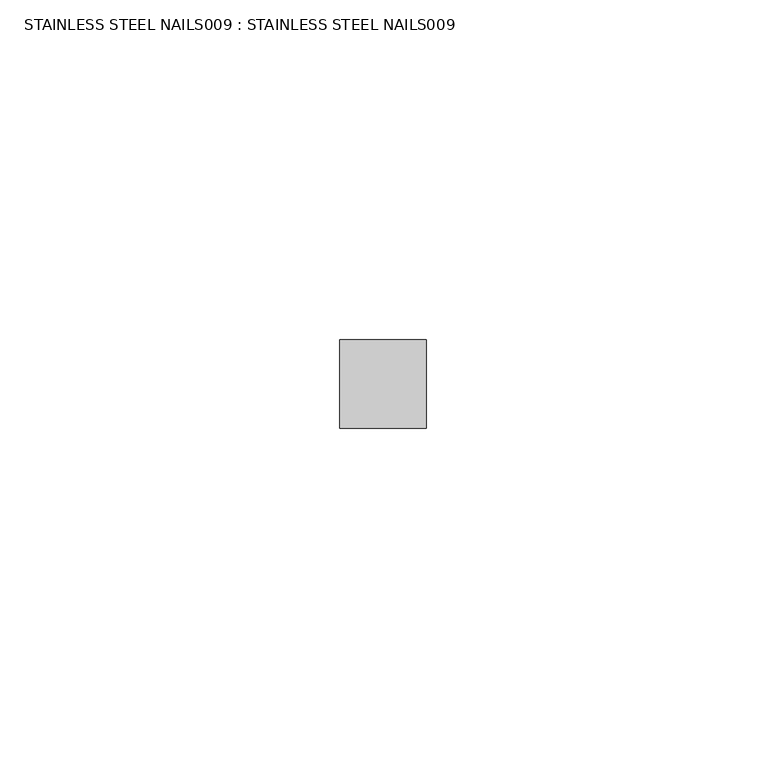
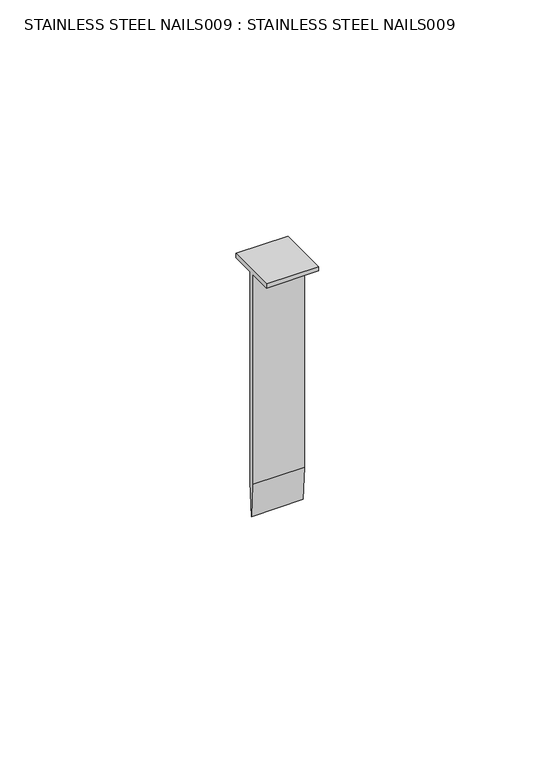
"""IFC4 building model written with IfcOpenShell, lengths in millimetres: proxy geometry, STAINLESS STEEL NAILS009 : STAINLESS STEEL NAILS009."""

import ifcopenshell
import ifcopenshell.guid

model = None  # the IFC model being written
_history = None  # IfcOwnerHistory: only IFC2X3 demands one
_inside = {}  # id of a spatial element -> (the spatial element, [elements in it])
_under = {}  # id of a project, library or spatial element -> (it, [spatial elements below it])
_declared = {}  # id of a project -> (the project, [libraries it declares])
_typed = {}  # id of a type object -> (the type object, [elements of that type])
_made_of = {}  # id of a material, layer set ... -> (it, [elements and type objects made of it])


def new_model(schema):
    """Start an empty IFC model of exactly this schema.

    Asked for "IFC4X3", IfcOpenShell would pick the latest addendum, in which some entities
    have other attributes; the version numbers below select the first issue.
    IFC2X3 requires an IfcOwnerHistory on every rooted entity: one is made here for all.
    """
    global model, _history
    if schema == "IFC4X3":
        model = ifcopenshell.file(schema_version=(4, 3, 0, 0))
    else:
        model = ifcopenshell.file(schema=schema)
    _inside.clear()
    _under.clear()
    _declared.clear()
    _typed.clear()
    _made_of.clear()
    _history = None
    if model.schema == "IFC2X3":
        org = make("IfcOrganization", Name="unknown")
        user = make(
            "IfcPersonAndOrganization",
            ThePerson=make("IfcPerson", FamilyName="unknown"),
            TheOrganization=org,
        )
        app = make(
            "IfcApplication",
            ApplicationDeveloper=org,
            Version="unknown",
            ApplicationFullName="unknown",
            ApplicationIdentifier="unknown",
        )
        _history = make(
            "IfcOwnerHistory",
            OwningUser=user,
            OwningApplication=app,
            ChangeAction="ADDED",
            CreationDate=0,
        )
    return model


def make(cls, **values):
    """One entity of the class cls with the attributes given. An attribute that is None is left unset."""
    return model.create_entity(
        cls, **{name: value for name, value in values.items() if value is not None}
    )


def rooted(cls, **values):
    """An entity with a GlobalId (a new one), such as an element, a storey or a relation."""
    return make(cls, GlobalId=ifcopenshell.guid.new(), OwnerHistory=_history, **values)


def si_unit(unit_type, name, prefix=None):
    """IfcSIUnit, for example si_unit("LENGTHUNIT", "METRE", prefix="MILLI")."""
    return make("IfcSIUnit", UnitType=unit_type, Prefix=prefix, Name=name)


def assignment(units):
    """IfcUnitAssignment: the units of a project."""
    return None if units is None else make("IfcUnitAssignment", Units=units)


def point(xyz):
    """IfcCartesianPoint."""
    return None if xyz is None else make("IfcCartesianPoint", Coordinates=xyz)


def direction(xyz):
    """IfcDirection."""
    return None if xyz is None else make("IfcDirection", DirectionRatios=xyz)


def frame(location, z_axis=None, x_axis=None):
    """IfcAxis2Placement3D, a coordinate frame: its origin and axes. An axis left out is left unset."""
    return make(
        "IfcAxis2Placement3D",
        Location=point(location),
        Axis=direction(z_axis),
        RefDirection=direction(x_axis),
    )


def origin():
    """The frame at (0, 0, 0) with its axes left unset."""
    return frame((0.0, 0.0, 0.0))


def place(relative_to, where):
    """IfcLocalPlacement: puts the frame where relative to a parent placement (None: the world)."""
    return make(
        "IfcLocalPlacement", PlacementRelTo=relative_to, RelativePlacement=where
    )


def context(
    kind, dimensions, precision=None, world=None, true_north=None, identifier=None
):
    """IfcGeometricRepresentationContext, for example the 3D "Model" context."""
    return make(
        "IfcGeometricRepresentationContext",
        ContextIdentifier=identifier,
        ContextType=kind,
        CoordinateSpaceDimension=dimensions,
        Precision=precision,
        WorldCoordinateSystem=world,
        TrueNorth=true_north,
    )


def project(units=None, contexts=None):
    """IfcProject with its units and contexts."""
    return rooted(
        "IfcProject",
        Name="project",
        RepresentationContexts=contexts,
        UnitsInContext=assignment(units),
    )


def spatial(cls, under=None, at=None, **own):
    """A site, building, storey or space (cls), placed at a placement, below another one or the project."""
    s = rooted(cls, ObjectPlacement=at, **own)
    if under is not None:
        _under.setdefault(under.id(), (under, []))[1].append(s)
    return s


def polyline(points):
    """IfcPolyline through the points."""
    return make("IfcPolyline", Points=[point(p) for p in points])


def outline(outer, holes=None, kind="AREA"):
    """IfcArbitraryClosedProfileDef: a profile drawn as a closed curve; with holes, ...WithVoids."""
    if holes is None:
        return make("IfcArbitraryClosedProfileDef", ProfileType=kind, OuterCurve=outer)
    return make(
        "IfcArbitraryProfileDefWithVoids",
        ProfileType=kind,
        OuterCurve=outer,
        InnerCurves=holes,
    )


def extrude(swept, where, along, depth):
    """IfcExtrudedAreaSolid: the profile swept, set in the frame where, extruded along a direction by depth."""
    return make(
        "IfcExtrudedAreaSolid",
        SweptArea=swept,
        Position=where,
        ExtrudedDirection=direction(along),
        Depth=depth,
    )


def shape(context_of_items, identifier, shape_type, items):
    """IfcShapeRepresentation: the items that make up one representation, for example the "Body"."""
    return make(
        "IfcShapeRepresentation",
        ContextOfItems=context_of_items,
        RepresentationIdentifier=identifier,
        RepresentationType=shape_type,
        Items=items,
    )


def source(mapping_origin, context_of_items, identifier, shape_type, items):
    """IfcRepresentationMap: a shape defined once, which mapped items show again and again."""
    return make(
        "IfcRepresentationMap",
        MappingOrigin=mapping_origin,
        MappedRepresentation=shape(context_of_items, identifier, shape_type, items),
    )


def transform(
    local_origin,
    x_axis=None,
    y_axis=None,
    z_axis=None,
    scale=None,
    scale2=None,
    scale3=None,
    uniform=True,
):
    """IfcCartesianTransformationOperator3D, or its non-uniform kind. x_axis, y_axis, z_axis: its Axis1, 2, 3."""
    if uniform:
        return make(
            "IfcCartesianTransformationOperator3D",
            Axis1=direction(x_axis),
            Axis2=direction(y_axis),
            LocalOrigin=point(local_origin),
            Scale=scale,
            Axis3=direction(z_axis),
        )
    return make(
        "IfcCartesianTransformationOperator3DnonUniform",
        Axis1=direction(x_axis),
        Axis2=direction(y_axis),
        LocalOrigin=point(local_origin),
        Scale=scale,
        Axis3=direction(z_axis),
        Scale2=scale2,
        Scale3=scale3,
    )


def mapped(mapping_source, mapping_target):
    """IfcMappedItem: shows the shape of a source again, moved by a transform."""
    return make(
        "IfcMappedItem", MappingSource=mapping_source, MappingTarget=mapping_target
    )


def made_of(thing, what):
    """Note that an element or type object is made of a material, layer set ...; save() writes the relation."""
    if what is not None:
        _made_of.setdefault(what.id(), (what, []))[1].append(thing)
    return thing


def element(
    cls,
    number,
    at=None,
    inside=None,
    cuts=None,
    type_object=None,
    material=None,
    context=None,
    identifier="Body",
    shape_type=None,
    held_by="IfcProductDefinitionShape",
    body=None,
    shapes=None,
    **own,
):
    """One element of the class cls, such as IfcWall. Its Tag is "e" and its number.

    at: its placement. inside: the storey or other place that contains it. cuts: it is an
    opening in that element (IfcRelVoidsElement). A single representation is given by context,
    identifier, shape_type and body (its items); several are given by shapes. held_by: the class
    of the entity that holds the representations. save() writes the other relations.
    """
    e = rooted(cls, Tag="e%d" % number, ObjectPlacement=at, **own)
    if body is not None:
        shapes = [shape(context, identifier, shape_type, body)]
    if shapes is not None:
        e.Representation = make(held_by, Representations=shapes)
    if inside is not None:
        _inside.setdefault(inside.id(), (inside, []))[1].append(e)
    if cuts is not None:
        rooted(
            "IfcRelVoidsElement", RelatingBuildingElement=cuts, RelatedOpeningElement=e
        )
    if type_object is not None:
        _typed.setdefault(type_object.id(), (type_object, []))[1].append(e)
    return made_of(e, material)


def aggregate(whole, parts):
    """IfcRelAggregates: a whole, such as a stair, and the parts it consists of."""
    return rooted("IfcRelAggregates", RelatingObject=whole, RelatedObjects=parts)


def save(model, path):
    """Write the relations noted so far, then the file.

    IfcRelAggregates (storeys below a building ...), IfcRelContainedInSpatialStructure (elements
    in a storey), IfcRelDefinesByType, IfcRelAssociatesMaterial and IfcRelDeclares: one each for
    every whole, place, type object, material and project.
    """
    for whole, parts in _under.values():
        aggregate(whole, parts)
    for where, things in _inside.values():
        rooted(
            "IfcRelContainedInSpatialStructure",
            RelatedElements=things,
            RelatingStructure=where,
        )
    for kind, things in _typed.values():
        rooted("IfcRelDefinesByType", RelatedObjects=things, RelatingType=kind)
    for what, things in _made_of.values():
        rooted("IfcRelAssociatesMaterial", RelatedObjects=things, RelatingMaterial=what)
    for by, libraries in _declared.values():
        rooted("IfcRelDeclares", RelatingContext=by, RelatedDefinitions=libraries)
    model.write(path)


def stainless_steel_nails009_stainless_steel_nails009_c75e95d3(model_context):
    return source(origin(), model_context, "Body", "SweptSolid", [
        extrude(outline(polyline([(-5490.4870231, 40241.4271837), (-5490.4870231, 40242.5103824), (-5477.4886393, 40242.5103824), (-5477.4886393, 40241.4271837), (-5483.4462319, 40241.4271837), (-5483.4462319, 40187.1010401), (-5483.9878312, 40178.4354508), (-5484.5294305, 40187.1010401), (-5484.5294305, 40241.4271837), (-5490.4870231, 40241.4271837)])), frame((14383.0178845, 0.0, 0.0), z_axis=(1.0, 0.0, 0.0), x_axis=(0.0, 1.0, 0.0)), (0.0, 0.0, 1.0), 12.7),
    ])


if __name__ == "__main__":
    model = new_model("IFC4")
    model_context = context("Model", 3, world=origin())
    ifc_project = project(units=[si_unit("LENGTHUNIT", "METRE", prefix="MILLI")], contexts=[model_context])
    site = spatial("IfcSite", under=ifc_project)
    building = spatial("IfcBuilding", under=site)
    placement = place(None, origin())
    stainless_steel_nails009_stainless_steel_nails009_shape = stainless_steel_nails009_stainless_steel_nails009_c75e95d3(model_context)
    element("IfcBuildingElementProxy", 1, Name="STAINLESS STEEL NAILS009 : STAINLESS STEEL NAILS009", ObjectType="STAINLESS STEEL NAILS009 : STAINLESS STEEL NAILS009", at=placement, inside=building, context=model_context, shape_type="MappedRepresentation", body=[
        mapped(stainless_steel_nails009_stainless_steel_nails009_shape, transform((0.0, 0.0, 0.0), x_axis=(1.0, 0.0, 0.0), y_axis=(0.0, 1.0, 0.0), z_axis=(0.0, 0.0, 1.0))),
    ])
    save(model, "model.ifc")

# Revit data of these elements
# Type "STAINLESS STEEL NAILS009 : STAINLESS STEEL NAILS009"
#   NameOverride = "STAINLESS STEEL NAILS009"
# Element 1 (IfcBuildingElementProxy, "STAINLESS STEEL NAILS009 : STAINLESS STEEL NAILS009")
#   Materials on its faces: "1 3/4\" STAINLESS STEEL RINGSHANK 5D COMMON NAILS @ 4\" (101.6MM) O.C. FIRESTONE PROVIDED MAX., 1/2\" STAGGERED"
# Materials
#   "1 3/4\" STAINLESS STEEL RINGSHANK 5D COMMON NAILS @ 4\" (101.6MM) O.C. FIRESTONE PROVIDED MAX., 1/2\" STAGGERED": class "Unassigned", colour RGB 255 255 255, transparency 0
